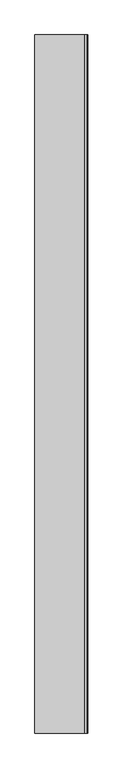
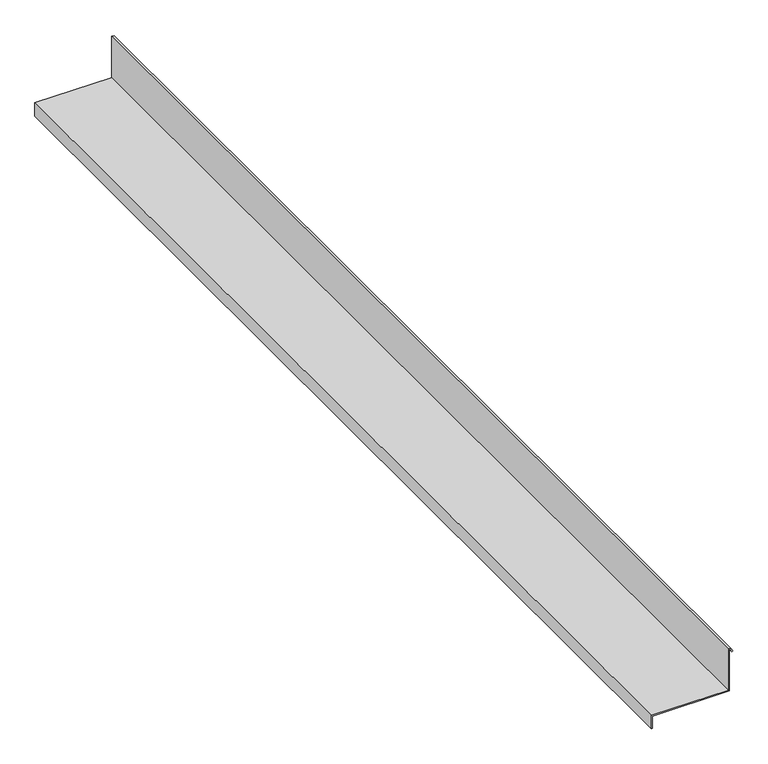
"""IFC4 building model written with IfcOpenShell, lengths in millimetres: proxy geometry, Flashing9:Flashing019:293133 : Flashing9:Flashing019:293133."""

from ifc_helpers import new_model, si_unit, frame, origin, place, context, project, spatial, polyline, outline, extrude, source, transform, mapped, element, save


def generic_models_d10c500d(model_context):
    return source(origin(), model_context, "Body", "SweptSolid", [
        extrude(outline(polyline([(40777.8359375, 21430.8020767), (40784.7382813, 21426.977858), (40784.7382813, 21422.2942642), (40703.2466161, 21422.2942642), (40703.2466161, 21278.852858), (40677.1179688, 21278.852858), (40677.1179688, 21280.852858), (40701.2466161, 21280.852858), (40701.2466161, 21424.2942642), (40782.7382813, 21424.2942642), (40782.7382813, 21425.7994973), (40776.8666698, 21429.0526425), (40777.8359375, 21430.8020767)])), frame((0.0, 8260.4774777, 0.0), z_axis=(0.0, 1.0, 0.0), x_axis=(0.0, 0.0, 1.0)), (0.0, 0.0, 1.0), 2000.0),
    ])


if __name__ == "__main__":
    model = new_model("IFC4")
    model_context = context("Model", 3, world=origin())
    ifc_project = project(units=[si_unit("LENGTHUNIT", "METRE", prefix="MILLI")], contexts=[model_context])
    site = spatial("IfcSite", under=ifc_project)
    building = spatial("IfcBuilding", under=site)
    placement = place(None, origin())
    generic_models_shape = generic_models_d10c500d(model_context)
    element("IfcBuildingElementProxy", 1, Name="Flashing9:Flashing019:293133 : Flashing9:Flashing019:293133", ObjectType="Flashing9:Flashing019:293133 : Flashing9:Flashing019:293133", at=placement, inside=building, context=model_context, shape_type="MappedRepresentation", body=[
        mapped(generic_models_shape, transform((0.0, 0.0, 0.0), x_axis=(1.0, 0.0, 0.0), y_axis=(0.0, 1.0, 0.0), z_axis=(0.0, 0.0, 1.0))),
    ])
    save(model, "model.ifc")

# Revit data of these elements
# Type "Flashing9:Flashing019:293133 : Flashing9:Flashing019:293133"
#   NameOverride = "Flashing9:Flashing019:293133"
#   ObjectTypeOverride = "Flashing9:Flashing019"
#   Reference = "Flashing019"
#   Category = "Generic Models"
#   Tag = "293133"
# Element 1 (IfcBuildingElementProxy, "Flashing9:Flashing019:293133 : Flashing9:Flashing019:293133")
#   Materials on its faces: "BRAKE METAL TO WRAP FRAMING OVER BITUTHANE"
# Materials
#   "BRAKE METAL TO WRAP FRAMING OVER BITUTHANE": class "Unassigned", colour RGB 128 128 128, transparency 0, Cost = 0
